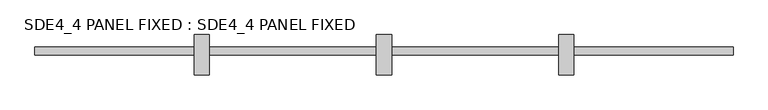
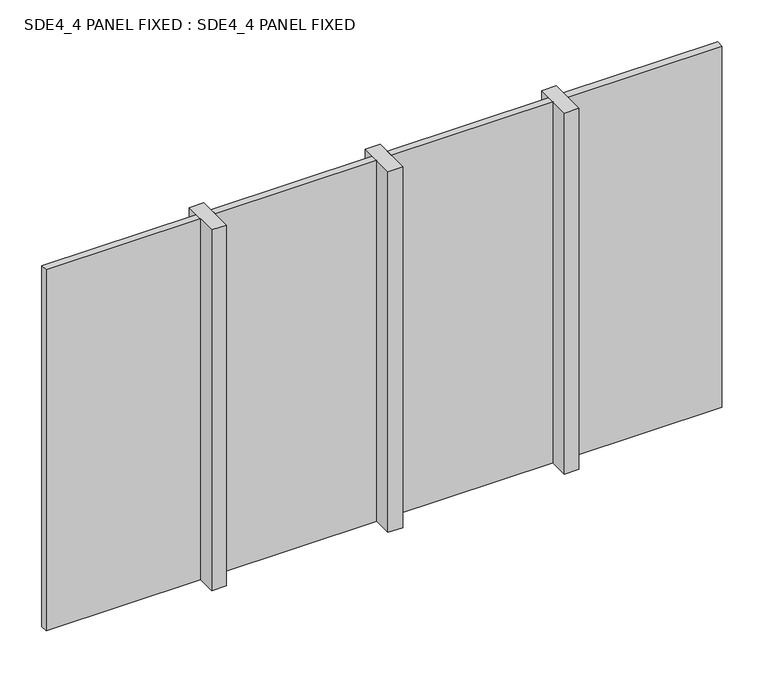
"""IFC4 building model written with IfcOpenShell, lengths in millimetres: plate geometry, SDE4_4 PANEL FIXED : SDE4_4 PANEL FIXED."""

import ifcopenshell
import ifcopenshell.guid

model = None  # the IFC model being written
_history = None  # IfcOwnerHistory: only IFC2X3 demands one
_inside = {}  # id of a spatial element -> (the spatial element, [elements in it])
_under = {}  # id of a project, library or spatial element -> (it, [spatial elements below it])
_declared = {}  # id of a project -> (the project, [libraries it declares])
_typed = {}  # id of a type object -> (the type object, [elements of that type])
_made_of = {}  # id of a material, layer set ... -> (it, [elements and type objects made of it])


def new_model(schema):
    """Start an empty IFC model of exactly this schema.

    Asked for "IFC4X3", IfcOpenShell would pick the latest addendum, in which some entities
    have other attributes; the version numbers below select the first issue.
    IFC2X3 requires an IfcOwnerHistory on every rooted entity: one is made here for all.
    """
    global model, _history
    if schema == "IFC4X3":
        model = ifcopenshell.file(schema_version=(4, 3, 0, 0))
    else:
        model = ifcopenshell.file(schema=schema)
    _inside.clear()
    _under.clear()
    _declared.clear()
    _typed.clear()
    _made_of.clear()
    _history = None
    if model.schema == "IFC2X3":
        org = make("IfcOrganization", Name="unknown")
        user = make(
            "IfcPersonAndOrganization",
            ThePerson=make("IfcPerson", FamilyName="unknown"),
            TheOrganization=org,
        )
        app = make(
            "IfcApplication",
            ApplicationDeveloper=org,
            Version="unknown",
            ApplicationFullName="unknown",
            ApplicationIdentifier="unknown",
        )
        _history = make(
            "IfcOwnerHistory",
            OwningUser=user,
            OwningApplication=app,
            ChangeAction="ADDED",
            CreationDate=0,
        )
    return model


def make(cls, **values):
    """One entity of the class cls with the attributes given. An attribute that is None is left unset."""
    return model.create_entity(
        cls, **{name: value for name, value in values.items() if value is not None}
    )


def rooted(cls, **values):
    """An entity with a GlobalId (a new one), such as an element, a storey or a relation."""
    return make(cls, GlobalId=ifcopenshell.guid.new(), OwnerHistory=_history, **values)


def si_unit(unit_type, name, prefix=None):
    """IfcSIUnit, for example si_unit("LENGTHUNIT", "METRE", prefix="MILLI")."""
    return make("IfcSIUnit", UnitType=unit_type, Prefix=prefix, Name=name)


def assignment(units):
    """IfcUnitAssignment: the units of a project."""
    return None if units is None else make("IfcUnitAssignment", Units=units)


def point(xyz):
    """IfcCartesianPoint."""
    return None if xyz is None else make("IfcCartesianPoint", Coordinates=xyz)


def direction(xyz):
    """IfcDirection."""
    return None if xyz is None else make("IfcDirection", DirectionRatios=xyz)


def frame(location, z_axis=None, x_axis=None):
    """IfcAxis2Placement3D, a coordinate frame: its origin and axes. An axis left out is left unset."""
    return make(
        "IfcAxis2Placement3D",
        Location=point(location),
        Axis=direction(z_axis),
        RefDirection=direction(x_axis),
    )


def origin():
    """The frame at (0, 0, 0) with its axes left unset."""
    return frame((0.0, 0.0, 0.0))


def origin_with_axes():
    """The frame at (0, 0, 0) with the z axis (0, 0, 1) and the x axis (1, 0, 0) written out."""
    return frame((0.0, 0.0, 0.0), z_axis=(0.0, 0.0, 1.0), x_axis=(1.0, 0.0, 0.0))


def place(relative_to, where):
    """IfcLocalPlacement: puts the frame where relative to a parent placement (None: the world)."""
    return make(
        "IfcLocalPlacement", PlacementRelTo=relative_to, RelativePlacement=where
    )


def context(
    kind, dimensions, precision=None, world=None, true_north=None, identifier=None
):
    """IfcGeometricRepresentationContext, for example the 3D "Model" context."""
    return make(
        "IfcGeometricRepresentationContext",
        ContextIdentifier=identifier,
        ContextType=kind,
        CoordinateSpaceDimension=dimensions,
        Precision=precision,
        WorldCoordinateSystem=world,
        TrueNorth=true_north,
    )


def project(units=None, contexts=None):
    """IfcProject with its units and contexts."""
    return rooted(
        "IfcProject",
        Name="project",
        RepresentationContexts=contexts,
        UnitsInContext=assignment(units),
    )


def spatial(cls, under=None, at=None, **own):
    """A site, building, storey or space (cls), placed at a placement, below another one or the project."""
    s = rooted(cls, ObjectPlacement=at, **own)
    if under is not None:
        _under.setdefault(under.id(), (under, []))[1].append(s)
    return s


def polyline(points):
    """IfcPolyline through the points."""
    return make("IfcPolyline", Points=[point(p) for p in points])


def outline(outer, holes=None, kind="AREA"):
    """IfcArbitraryClosedProfileDef: a profile drawn as a closed curve; with holes, ...WithVoids."""
    if holes is None:
        return make("IfcArbitraryClosedProfileDef", ProfileType=kind, OuterCurve=outer)
    return make(
        "IfcArbitraryProfileDefWithVoids",
        ProfileType=kind,
        OuterCurve=outer,
        InnerCurves=holes,
    )


def extrude(swept, where, along, depth):
    """IfcExtrudedAreaSolid: the profile swept, set in the frame where, extruded along a direction by depth."""
    return make(
        "IfcExtrudedAreaSolid",
        SweptArea=swept,
        Position=where,
        ExtrudedDirection=direction(along),
        Depth=depth,
    )


def shape(context_of_items, identifier, shape_type, items):
    """IfcShapeRepresentation: the items that make up one representation, for example the "Body"."""
    return make(
        "IfcShapeRepresentation",
        ContextOfItems=context_of_items,
        RepresentationIdentifier=identifier,
        RepresentationType=shape_type,
        Items=items,
    )


def source(mapping_origin, context_of_items, identifier, shape_type, items):
    """IfcRepresentationMap: a shape defined once, which mapped items show again and again."""
    return make(
        "IfcRepresentationMap",
        MappingOrigin=mapping_origin,
        MappedRepresentation=shape(context_of_items, identifier, shape_type, items),
    )


def transform(
    local_origin,
    x_axis=None,
    y_axis=None,
    z_axis=None,
    scale=None,
    scale2=None,
    scale3=None,
    uniform=True,
):
    """IfcCartesianTransformationOperator3D, or its non-uniform kind. x_axis, y_axis, z_axis: its Axis1, 2, 3."""
    if uniform:
        return make(
            "IfcCartesianTransformationOperator3D",
            Axis1=direction(x_axis),
            Axis2=direction(y_axis),
            LocalOrigin=point(local_origin),
            Scale=scale,
            Axis3=direction(z_axis),
        )
    return make(
        "IfcCartesianTransformationOperator3DnonUniform",
        Axis1=direction(x_axis),
        Axis2=direction(y_axis),
        LocalOrigin=point(local_origin),
        Scale=scale,
        Axis3=direction(z_axis),
        Scale2=scale2,
        Scale3=scale3,
    )


def mapped(mapping_source, mapping_target):
    """IfcMappedItem: shows the shape of a source again, moved by a transform."""
    return make(
        "IfcMappedItem", MappingSource=mapping_source, MappingTarget=mapping_target
    )


def made_of(thing, what):
    """Note that an element or type object is made of a material, layer set ...; save() writes the relation."""
    if what is not None:
        _made_of.setdefault(what.id(), (what, []))[1].append(thing)
    return thing


def element(
    cls,
    number,
    at=None,
    inside=None,
    cuts=None,
    type_object=None,
    material=None,
    context=None,
    identifier="Body",
    shape_type=None,
    held_by="IfcProductDefinitionShape",
    body=None,
    shapes=None,
    **own,
):
    """One element of the class cls, such as IfcWall. Its Tag is "e" and its number.

    at: its placement. inside: the storey or other place that contains it. cuts: it is an
    opening in that element (IfcRelVoidsElement). A single representation is given by context,
    identifier, shape_type and body (its items); several are given by shapes. held_by: the class
    of the entity that holds the representations. save() writes the other relations.
    """
    e = rooted(cls, Tag="e%d" % number, ObjectPlacement=at, **own)
    if body is not None:
        shapes = [shape(context, identifier, shape_type, body)]
    if shapes is not None:
        e.Representation = make(held_by, Representations=shapes)
    if inside is not None:
        _inside.setdefault(inside.id(), (inside, []))[1].append(e)
    if cuts is not None:
        rooted(
            "IfcRelVoidsElement", RelatingBuildingElement=cuts, RelatedOpeningElement=e
        )
    if type_object is not None:
        _typed.setdefault(type_object.id(), (type_object, []))[1].append(e)
    return made_of(e, material)


def aggregate(whole, parts):
    """IfcRelAggregates: a whole, such as a stair, and the parts it consists of."""
    return rooted("IfcRelAggregates", RelatingObject=whole, RelatedObjects=parts)


def save(model, path):
    """Write the relations noted so far, then the file.

    IfcRelAggregates (storeys below a building ...), IfcRelContainedInSpatialStructure (elements
    in a storey), IfcRelDefinesByType, IfcRelAssociatesMaterial and IfcRelDeclares: one each for
    every whole, place, type object, material and project.
    """
    for whole, parts in _under.values():
        aggregate(whole, parts)
    for where, things in _inside.values():
        rooted(
            "IfcRelContainedInSpatialStructure",
            RelatedElements=things,
            RelatingStructure=where,
        )
    for kind, things in _typed.values():
        rooted("IfcRelDefinesByType", RelatedObjects=things, RelatingType=kind)
    for what, things in _made_of.values():
        rooted("IfcRelAssociatesMaterial", RelatedObjects=things, RelatingMaterial=what)
    for by, libraries in _declared.values():
        rooted("IfcRelDeclares", RelatingContext=by, RelatedDefinitions=libraries)
    model.write(path)


def sde4_4_panel_fixed_sde4_4_panel_fixed_2c311422(model_context):
    return source(origin(), model_context, "Body", "SweptSolid", [
        extrude(outline(polyline([(-1150.0, 132.5), (-1150.0, -132.5), (-1250.0, -132.5), (-1250.0, 132.5), (-1150.0, 132.5)])), origin_with_axes(), (0.0, 0.0, 1.0), 2597.1714687),
        extrude(outline(polyline([(50.0, 132.5), (50.0, -132.5), (-50.0, -132.5), (-50.0, 132.5), (50.0, 132.5)])), origin_with_axes(), (0.0, 0.0, 1.0), 2597.1714687),
        extrude(outline(polyline([(1250.0, 132.5), (1250.0, -132.5), (1150.0, -132.5), (1150.0, 132.5), (1250.0, 132.5)])), origin_with_axes(), (0.0, 0.0, 1.0), 2597.1714687),
        extrude(outline(polyline([(2299.0, 50.0), (2299.0, 0.0), (1250.0, 0.0), (1250.0, 50.0), (2299.0, 50.0)])), origin_with_axes(), (0.0, 0.0, 1.0), 2597.1714687),
        extrude(outline(polyline([(1150.0, 50.0), (1150.0, 0.0), (50.0, 0.0), (50.0, 50.0), (1150.0, 50.0)])), origin_with_axes(), (0.0, 0.0, 1.0), 2597.1714687),
        extrude(outline(polyline([(-50.0, 50.0), (-50.0, 0.0), (-1150.0, 0.0), (-1150.0, 50.0), (-50.0, 50.0)])), origin_with_axes(), (0.0, 0.0, 1.0), 2597.1714687),
        extrude(outline(polyline([(-1250.0, 50.0), (-1250.0, 0.0), (-2300.0, 0.0), (-2300.0, 50.0), (-1250.0, 50.0)])), origin_with_axes(), (0.0, 0.0, 1.0), 2597.1714687),
    ])


if __name__ == "__main__":
    model = new_model("IFC4")
    model_context = context("Model", 3, world=origin())
    ifc_project = project(units=[si_unit("LENGTHUNIT", "METRE", prefix="MILLI")], contexts=[model_context])
    site = spatial("IfcSite", under=ifc_project)
    building = spatial("IfcBuilding", under=site)
    placement = place(None, origin())
    sde4_4_panel_fixed_sde4_4_panel_fixed_shape = sde4_4_panel_fixed_sde4_4_panel_fixed_2c311422(model_context)
    element("IfcPlate", 1, ObjectType="SDE4_4 PANEL FIXED : SDE4_4 PANEL FIXED", at=placement, inside=building, context=model_context, shape_type="MappedRepresentation", body=[
        mapped(sde4_4_panel_fixed_sde4_4_panel_fixed_shape, transform((0.0, 0.0, 0.0), x_axis=(1.0, 0.0, 0.0), y_axis=(0.0, 1.0, 0.0), z_axis=(0.0, 0.0, 1.0))),
    ])
    save(model, "model.ifc")

# Revit data of these elements
# Type "SDE4_4 PANEL FIXED : SDE4_4 PANEL FIXED"
#   Type Mark = "CW-GLASS"
#   Analytic Construction = "<None>"
#   Glass = Glass
#   Frame = Aluminium
# Element 1 (IfcPlate, "SDE4_4 PANEL FIXED : SDE4_4 PANEL FIXED")
#   Materials on its faces: "Glass", "Aluminium"
# Materials
#   "Glass": class "Glass", colour RGB 0 128 192, transparency 0.9, Keynote = "L40", Cost = 0
#   "Aluminium": class "Unassigned", colour RGB 247 247 247, transparency 0, Cost = 0
